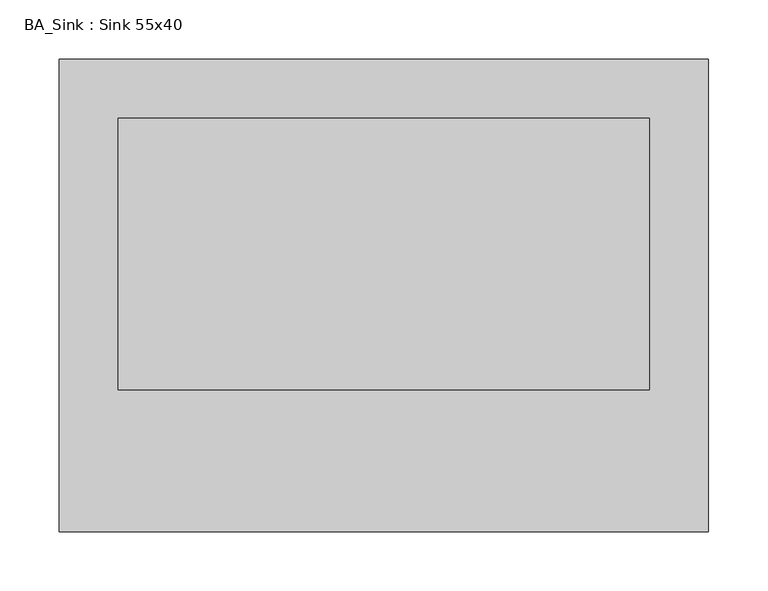
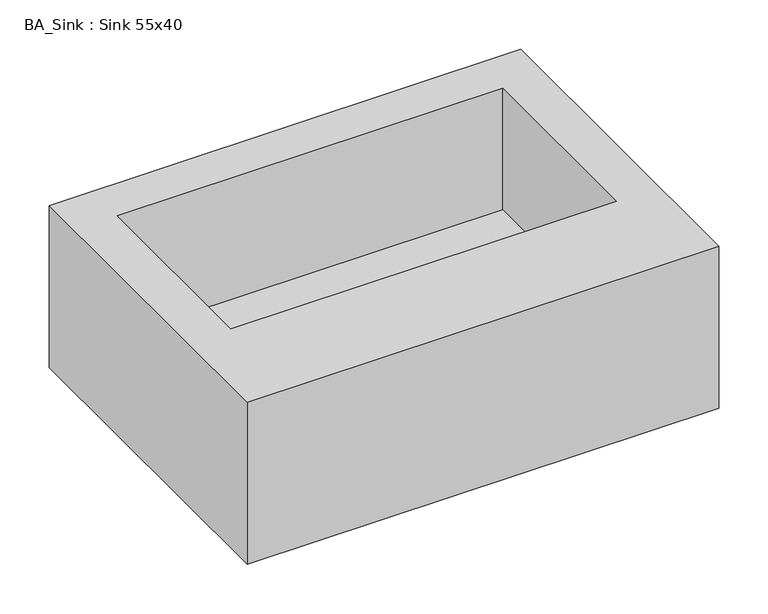
"""IFC4 building model written with IfcOpenShell, lengths in millimetres: flow terminal geometry, BA_Sink : Sink 55x40."""

import ifcopenshell
import ifcopenshell.guid

model = None  # the IFC model being written
_history = None  # IfcOwnerHistory: only IFC2X3 demands one
_inside = {}  # id of a spatial element -> (the spatial element, [elements in it])
_under = {}  # id of a project, library or spatial element -> (it, [spatial elements below it])
_declared = {}  # id of a project -> (the project, [libraries it declares])
_typed = {}  # id of a type object -> (the type object, [elements of that type])
_made_of = {}  # id of a material, layer set ... -> (it, [elements and type objects made of it])


def new_model(schema):
    """Start an empty IFC model of exactly this schema.

    Asked for "IFC4X3", IfcOpenShell would pick the latest addendum, in which some entities
    have other attributes; the version numbers below select the first issue.
    IFC2X3 requires an IfcOwnerHistory on every rooted entity: one is made here for all.
    """
    global model, _history
    if schema == "IFC4X3":
        model = ifcopenshell.file(schema_version=(4, 3, 0, 0))
    else:
        model = ifcopenshell.file(schema=schema)
    _inside.clear()
    _under.clear()
    _declared.clear()
    _typed.clear()
    _made_of.clear()
    _history = None
    if model.schema == "IFC2X3":
        org = make("IfcOrganization", Name="unknown")
        user = make(
            "IfcPersonAndOrganization",
            ThePerson=make("IfcPerson", FamilyName="unknown"),
            TheOrganization=org,
        )
        app = make(
            "IfcApplication",
            ApplicationDeveloper=org,
            Version="unknown",
            ApplicationFullName="unknown",
            ApplicationIdentifier="unknown",
        )
        _history = make(
            "IfcOwnerHistory",
            OwningUser=user,
            OwningApplication=app,
            ChangeAction="ADDED",
            CreationDate=0,
        )
    return model


def make(cls, **values):
    """One entity of the class cls with the attributes given. An attribute that is None is left unset."""
    return model.create_entity(
        cls, **{name: value for name, value in values.items() if value is not None}
    )


def rooted(cls, **values):
    """An entity with a GlobalId (a new one), such as an element, a storey or a relation."""
    return make(cls, GlobalId=ifcopenshell.guid.new(), OwnerHistory=_history, **values)


def si_unit(unit_type, name, prefix=None):
    """IfcSIUnit, for example si_unit("LENGTHUNIT", "METRE", prefix="MILLI")."""
    return make("IfcSIUnit", UnitType=unit_type, Prefix=prefix, Name=name)


def assignment(units):
    """IfcUnitAssignment: the units of a project."""
    return None if units is None else make("IfcUnitAssignment", Units=units)


def point(xyz):
    """IfcCartesianPoint."""
    return None if xyz is None else make("IfcCartesianPoint", Coordinates=xyz)


def direction(xyz):
    """IfcDirection."""
    return None if xyz is None else make("IfcDirection", DirectionRatios=xyz)


def frame(location, z_axis=None, x_axis=None):
    """IfcAxis2Placement3D, a coordinate frame: its origin and axes. An axis left out is left unset."""
    return make(
        "IfcAxis2Placement3D",
        Location=point(location),
        Axis=direction(z_axis),
        RefDirection=direction(x_axis),
    )


def origin():
    """The frame at (0, 0, 0) with its axes left unset."""
    return frame((0.0, 0.0, 0.0))


def place(relative_to, where):
    """IfcLocalPlacement: puts the frame where relative to a parent placement (None: the world)."""
    return make(
        "IfcLocalPlacement", PlacementRelTo=relative_to, RelativePlacement=where
    )


def context(
    kind, dimensions, precision=None, world=None, true_north=None, identifier=None
):
    """IfcGeometricRepresentationContext, for example the 3D "Model" context."""
    return make(
        "IfcGeometricRepresentationContext",
        ContextIdentifier=identifier,
        ContextType=kind,
        CoordinateSpaceDimension=dimensions,
        Precision=precision,
        WorldCoordinateSystem=world,
        TrueNorth=true_north,
    )


def project(units=None, contexts=None):
    """IfcProject with its units and contexts."""
    return rooted(
        "IfcProject",
        Name="project",
        RepresentationContexts=contexts,
        UnitsInContext=assignment(units),
    )


def spatial(cls, under=None, at=None, **own):
    """A site, building, storey or space (cls), placed at a placement, below another one or the project."""
    s = rooted(cls, ObjectPlacement=at, **own)
    if under is not None:
        _under.setdefault(under.id(), (under, []))[1].append(s)
    return s


def faces_of(points, faces, orient=None, outer=None):
    """IfcFace entities. A face is a list of loops; a loop is a list of indices into points, from 0.

    orient and outer hold one flag for each loop. By default every Orientation is true, the
    first loop of a face is its IfcFaceOuterBound and the others are IfcFaceBound.
    """
    made = []
    for i, loops in enumerate(faces):
        bounds = []
        for j, loop in enumerate(loops):
            is_outer = j == 0 if outer is None else outer[i][j]
            bounds.append(
                make(
                    "IfcFaceOuterBound" if is_outer else "IfcFaceBound",
                    Bound=make("IfcPolyLoop", Polygon=[points[k] for k in loop]),
                    Orientation=True if orient is None else orient[i][j],
                )
            )
        made.append(make("IfcFace", Bounds=bounds))
    return made


def faceted_brep(points, faces, orient=None, outer=None, voids=None):
    """IfcFacetedBrep: a solid bounded by flat faces; with voids (closed shells), ...WithVoids."""
    shared = [point(p) for p in points]
    hull = make("IfcClosedShell", CfsFaces=faces_of(shared, faces, orient, outer))
    if voids is None:
        return make("IfcFacetedBrep", Outer=hull)
    return make(
        "IfcFacetedBrepWithVoids",
        Outer=hull,
        Voids=[
            make(cls, CfsFaces=faces_of(shared, fs, o, b)) for cls, fs, o, b in voids
        ],
    )


def shape(context_of_items, identifier, shape_type, items):
    """IfcShapeRepresentation: the items that make up one representation, for example the "Body"."""
    return make(
        "IfcShapeRepresentation",
        ContextOfItems=context_of_items,
        RepresentationIdentifier=identifier,
        RepresentationType=shape_type,
        Items=items,
    )


def source(mapping_origin, context_of_items, identifier, shape_type, items):
    """IfcRepresentationMap: a shape defined once, which mapped items show again and again."""
    return make(
        "IfcRepresentationMap",
        MappingOrigin=mapping_origin,
        MappedRepresentation=shape(context_of_items, identifier, shape_type, items),
    )


def transform(
    local_origin,
    x_axis=None,
    y_axis=None,
    z_axis=None,
    scale=None,
    scale2=None,
    scale3=None,
    uniform=True,
):
    """IfcCartesianTransformationOperator3D, or its non-uniform kind. x_axis, y_axis, z_axis: its Axis1, 2, 3."""
    if uniform:
        return make(
            "IfcCartesianTransformationOperator3D",
            Axis1=direction(x_axis),
            Axis2=direction(y_axis),
            LocalOrigin=point(local_origin),
            Scale=scale,
            Axis3=direction(z_axis),
        )
    return make(
        "IfcCartesianTransformationOperator3DnonUniform",
        Axis1=direction(x_axis),
        Axis2=direction(y_axis),
        LocalOrigin=point(local_origin),
        Scale=scale,
        Axis3=direction(z_axis),
        Scale2=scale2,
        Scale3=scale3,
    )


def mapped(mapping_source, mapping_target):
    """IfcMappedItem: shows the shape of a source again, moved by a transform."""
    return make(
        "IfcMappedItem", MappingSource=mapping_source, MappingTarget=mapping_target
    )


def made_of(thing, what):
    """Note that an element or type object is made of a material, layer set ...; save() writes the relation."""
    if what is not None:
        _made_of.setdefault(what.id(), (what, []))[1].append(thing)
    return thing


def element(
    cls,
    number,
    at=None,
    inside=None,
    cuts=None,
    type_object=None,
    material=None,
    context=None,
    identifier="Body",
    shape_type=None,
    held_by="IfcProductDefinitionShape",
    body=None,
    shapes=None,
    **own,
):
    """One element of the class cls, such as IfcWall. Its Tag is "e" and its number.

    at: its placement. inside: the storey or other place that contains it. cuts: it is an
    opening in that element (IfcRelVoidsElement). A single representation is given by context,
    identifier, shape_type and body (its items); several are given by shapes. held_by: the class
    of the entity that holds the representations. save() writes the other relations.
    """
    e = rooted(cls, Tag="e%d" % number, ObjectPlacement=at, **own)
    if body is not None:
        shapes = [shape(context, identifier, shape_type, body)]
    if shapes is not None:
        e.Representation = make(held_by, Representations=shapes)
    if inside is not None:
        _inside.setdefault(inside.id(), (inside, []))[1].append(e)
    if cuts is not None:
        rooted(
            "IfcRelVoidsElement", RelatingBuildingElement=cuts, RelatedOpeningElement=e
        )
    if type_object is not None:
        _typed.setdefault(type_object.id(), (type_object, []))[1].append(e)
    return made_of(e, material)


def aggregate(whole, parts):
    """IfcRelAggregates: a whole, such as a stair, and the parts it consists of."""
    return rooted("IfcRelAggregates", RelatingObject=whole, RelatedObjects=parts)


def save(model, path):
    """Write the relations noted so far, then the file.

    IfcRelAggregates (storeys below a building ...), IfcRelContainedInSpatialStructure (elements
    in a storey), IfcRelDefinesByType, IfcRelAssociatesMaterial and IfcRelDeclares: one each for
    every whole, place, type object, material and project.
    """
    for whole, parts in _under.values():
        aggregate(whole, parts)
    for where, things in _inside.values():
        rooted(
            "IfcRelContainedInSpatialStructure",
            RelatedElements=things,
            RelatingStructure=where,
        )
    for kind, things in _typed.values():
        rooted("IfcRelDefinesByType", RelatedObjects=things, RelatingType=kind)
    for what, things in _made_of.values():
        rooted("IfcRelAssociatesMaterial", RelatedObjects=things, RelatingMaterial=what)
    for by, libraries in _declared.values():
        rooted("IfcRelDeclares", RelatingContext=by, RelatedDefinitions=libraries)
    model.write(path)


def ba_sink_sink_55x40_4eaba232(model_context):
    return source(origin(), model_context, "Body", "Brep", [
        faceted_brep([(400.0, 475.0, 900.0), (-150.0, 475.0, 900.0), (-150.0, 75.0, 900.0), (400.0, 75.0, 900.0), (-100.0, 425.0, 900.0), (350.0, 425.0, 900.0), (350.0, 195.0, 900.0), (-100.0, 195.0, 900.0), (400.0, 475.0, 700.0), (400.0, 75.0, 700.0), (-150.0, 75.0, 700.0), (-150.0, 475.0, 700.0), (350.0, 425.0, 750.0), (-100.0, 425.0, 750.0), (-100.0, 195.0, 750.0), (350.0, 195.0, 750.0)], [[[0, 1, 2, 3], [4, 5, 6, 7]], [[8, 9, 10, 11]], [[1, 0, 8, 11]], [[2, 1, 11, 10]], [[3, 2, 10, 9]], [[0, 3, 9, 8]], [[12, 13, 14, 15]], [[13, 12, 5, 4]], [[14, 13, 4, 7]], [[15, 14, 7, 6]], [[12, 15, 6, 5]]]),
    ])


if __name__ == "__main__":
    model = new_model("IFC4")
    model_context = context("Model", 3, world=origin())
    ifc_project = project(units=[si_unit("LENGTHUNIT", "METRE", prefix="MILLI")], contexts=[model_context])
    site = spatial("IfcSite", under=ifc_project)
    building = spatial("IfcBuilding", under=site)
    placement = place(None, origin())
    ba_sink_sink_55x40_shape = ba_sink_sink_55x40_4eaba232(model_context)
    element("IfcFlowTerminal", 1, ObjectType="BA_Sink : Sink 55x40", at=placement, inside=building, context=model_context, shape_type="MappedRepresentation", body=[
        mapped(ba_sink_sink_55x40_shape, transform((0.0, 0.0, 0.0), x_axis=(1.0, 0.0, 0.0), y_axis=(0.0, 1.0, 0.0), z_axis=(0.0, 0.0, 1.0))),
    ])
    save(model, "model.ifc")

# Revit data of these elements
# Type "BA_Sink : Sink 55x40"
#   height = 900 mm
#   width = 550 mm
#   depth = 400 mm
#   Default Elevation = 0
# Element 1 (IfcFlowTerminal, "BA_Sink : Sink 55x40")
#   Materials on its faces: "Default"
# Materials
#   "Default": class "Generic", colour RGB 255 255 255, transparency 0, Cost = 0
